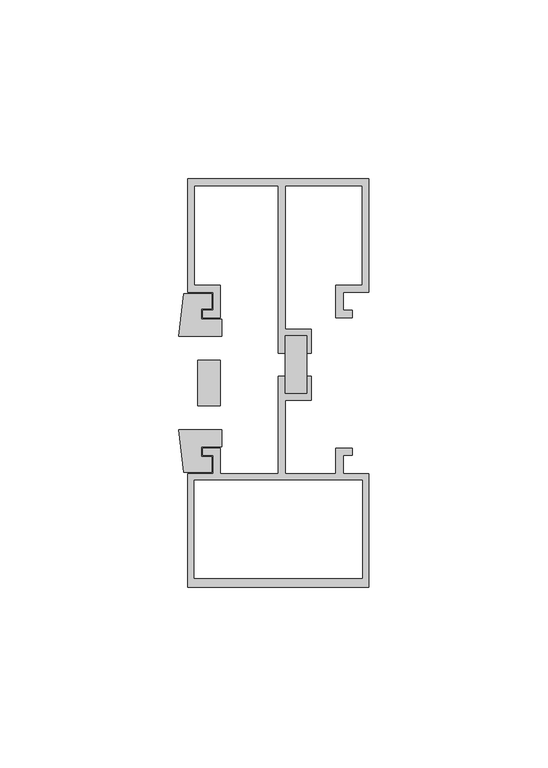
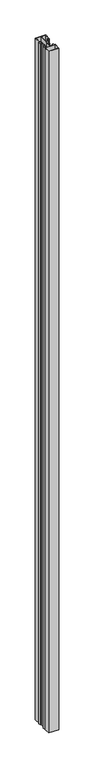
"""IFC4 building model written with IfcOpenShell, lengths in millimetres: proxy geometry, Generic Models 3:Generic Models 1:5:Generic Models 1:5 : Generic Models 3:Generic Models 1:300625:345888:Generic Models 1:5:Generic Models 1:5 : Generic Models 3:Generic Models 1:300625:345888 : Generic Models 3:Generic Models 1:5:Generic Models 1:5 : Generic Models 3:Generic Models 1:300625:345888:4 : Generic Models 3:Generic Models 1:5:Generic Models 1:5 : Generic Models 3:Generic Models 1:300625:345888:Generic Models 1:5:Generic Models 1:5 : Generic Models 3:Generic Models 1:300625:345888 : Generic Models 3:Generic Models 1:5:Generic Models 1:5 : Generic Models 3:Generic Models 1:300625:345888:301574."""

from ifc_helpers import new_model, si_unit, frame, origin, place, context, project, spatial, polyline, outline, extrude, source, transform, mapped, element, save


def generic_models_e0ac1aa3(model_context):
    return source(origin(), model_context, "Body", "SweptSolid", [
        extrude(outline(polyline([(570422.8035457, -579063.9802804), (570422.8035457, -579047.8688442), (570428.883333, -579047.8688442), (570428.883333, -579063.9802804), (570422.8035457, -579063.9802804)])), frame((0.0, 0.0, 66.3122056), z_axis=(0.0, 0.0, 1.0), x_axis=(1.0, 0.0, 0.0)), (0.0, 0.0, 1.0), 3584.971571),
        extrude(outline(polyline([(570398.3726303, -579067.3663841), (570398.3726303, -579054.6663841), (570404.7161787, -579054.6663841), (570404.7161787, -579067.3663841), (570398.3726303, -579067.3663841)])), frame((0.0, 0.0, 66.3122056), z_axis=(0.0, 0.0, 1.0), x_axis=(1.0, 0.0, 0.0)), (0.0, 0.0, 1.0), 3584.971571),
        extrude(outline(polyline([(570399.3995131, -579078.8588708), (570399.3995131, -579081.704549), (570402.3433729, -579081.704549), (570402.3433729, -579086.0026208), (570394.5036635, -579086.0026208), (570393.0427966, -579074.1048149), (570405.1130537, -579074.1048149), (570405.1130537, -579078.8588708), (570399.3995131, -579078.8588708)])), frame((0.0, 0.0, 66.3122056), z_axis=(0.0, 0.0, 1.0), x_axis=(1.0, 0.0, 0.0)), (0.0, 0.0, 1.0), 3584.971571),
        extrude(outline(polyline([(570394.5036635, -579036.0301474), (570402.3433729, -579036.0301474), (570402.3433729, -579040.3282192), (570399.3995131, -579040.3282192), (570399.3995131, -579043.1738974), (570405.1130537, -579043.1738974), (570405.1130537, -579047.9279532), (570393.0427966, -579047.9279532), (570394.5036635, -579036.0301474)])), frame((0.0, 0.0, 66.3122056), z_axis=(0.0, 0.0, 1.0), x_axis=(1.0, 0.0, 0.0)), (0.0, 0.0, 1.0), 3584.9377944),
        extrude(outline(polyline([(570446.2867239, -579118.1663841), (570395.5205005, -579118.1663841), (570395.5205005, -579086.3994958), (570402.7402479, -579086.3994958), (570402.7402479, -579081.307674), (570399.7963881, -579081.307674), (570399.7963881, -579079.2557458), (570404.7161787, -579079.2557458), (570404.7161787, -579086.3994958), (570420.9036122, -579086.3994958), (570420.9036122, -579059.1164506), (570422.8035457, -579059.1164506), (570422.8035457, -579063.9802804), (570428.883333, -579063.9802804), (570428.883333, -579059.1164506), (570430.1752878, -579059.1164506), (570430.1752878, -579065.8802139), (570422.8035457, -579065.8802139), (570422.8035457, -579086.3994958), (570437.0150484, -579086.3994958), (570437.0150484, -579079.2557458), (570441.586208, -579079.2557458), (570441.586208, -579081.307674), (570439.0669766, -579081.307674), (570439.0669766, -579086.3994958), (570446.2867239, -579086.3994958), (570446.2867239, -579118.1663841)]), holes=[polyline([(570397.420434, -579088.2994293), (570397.420434, -579115.6584719), (570444.3867904, -579115.6584719), (570444.3867904, -579088.2994293), (570397.420434, -579088.2994293)])]), frame((0.0, 0.0, 66.3122056), z_axis=(0.0, 0.0, 1.0), x_axis=(1.0, 0.0, 0.0)), (0.0, 0.0, 1.0), 3584.971571),
        extrude(outline(polyline([(570399.7963881, -579040.7250942), (570402.7402479, -579040.7250942), (570402.7402479, -579035.6332724), (570395.5205005, -579035.6332724), (570395.5205005, -579003.8663841), (570446.2867239, -579003.8663841), (570446.2867239, -579035.6332724), (570439.0669766, -579035.6332724), (570439.0669766, -579040.7250942), (570441.586208, -579040.7250942), (570441.586208, -579042.7770224), (570437.0150484, -579042.7770224), (570437.0150484, -579033.7333389), (570444.3645113, -579033.7333389), (570444.3645113, -579005.8423149), (570422.8035457, -579005.8423149), (570422.8035457, -579045.9689107), (570430.1752878, -579045.9689107), (570430.1752878, -579052.732674), (570428.883333, -579052.732674), (570428.883333, -579047.8688442), (570422.8035457, -579047.8688442), (570422.8035457, -579052.732674), (570420.9036122, -579052.732674), (570420.9036122, -579005.8423149), (570397.4302996, -579005.8423149), (570397.4302996, -579033.7333389), (570404.7161787, -579033.7333389), (570404.7161787, -579042.7770224), (570399.7963881, -579042.7770224), (570399.7963881, -579040.7250942)])), frame((0.0, 0.0, 66.3122056), z_axis=(0.0, 0.0, 1.0), x_axis=(1.0, 0.0, 0.0)), (0.0, 0.0, 1.0), 3584.971571),
    ])


if __name__ == "__main__":
    model = new_model("IFC4")
    model_context = context("Model", 3, world=origin())
    ifc_project = project(units=[si_unit("LENGTHUNIT", "METRE", prefix="MILLI")], contexts=[model_context])
    site = spatial("IfcSite", under=ifc_project)
    building = spatial("IfcBuilding", under=site)
    placement = place(None, origin())
    generic_models_shape = generic_models_e0ac1aa3(model_context)
    element("IfcBuildingElementProxy", 1, Name="Generic Models 3:Generic Models 1:5:Generic Models 1:5 : Generic Models 3:Generic Models 1:300625:345888:Generic Models 1:5:Generic Models 1:5 : Generic Models 3:Generic Models 1:300625:345888 : Generic Models 3:Generic Models 1:5:Generic Models 1:5 : Generic Models 3:Generic Models 1:300625:345888:4 : Generic Models 3:Generic Models 1:5:Generic Models 1:5 : Generic Models 3:Generic Models 1:300625:345888:Generic Models 1:5:Generic Models 1:5 : Generic Models 3:Generic Models 1:300625:345888 : Generic Models 3:Generic Models 1:5:Generic Models 1:5 : Generic Models 3:Generic Models 1:300625:345888:301574", ObjectType="Generic Models 3:Generic Models 1:5:Generic Models 1:5 : Generic Models 3:Generic Models 1:300625:345888:Generic Models 1:5:Generic Models 1:5 : Generic Models 3:Generic Models 1:300625:345888 : Generic Models 3:Generic Models 1:5:Generic Models 1:5 : Generic Models 3:Generic Models 1:300625:345888:4 : Generic Models 3:Generic Models 1:5:Generic Models 1:5 : Generic Models 3:Generic Models 1:300625:345888:Generic Models 1:5:Generic Models 1:5 : Generic Models 3:Generic Models 1:300625:345888 : Generic Models 3:Generic Models 1:5:Generic Models 1:5 : Generic Models 3:Generic Models 1:300625:345888:301574", at=placement, inside=building, context=model_context, shape_type="MappedRepresentation", body=[
        mapped(generic_models_shape, transform((0.0, 0.0, 0.0), x_axis=(1.0, 0.0, 0.0), y_axis=(0.0, 1.0, 0.0), z_axis=(0.0, 0.0, 1.0))),
    ])
    save(model, "model.ifc")

# Revit data of these elements
# Type "Generic Models 3:Generic Models 1:5:Generic Models 1:5 : Generic Models 3:Generic Models 1:300625:345888:Generic Models 1:5:Generic Models 1:5 : Generic Models 3:Generic Models 1:300625:345888 : Generic Models 3:Generic Models 1:5:Generic Models 1:5 : Generic Models 3:Generic Models 1:300625:345888:4 : Generic Models 3:Generic Models 1:5:Generic Models 1:5 : Generic Models 3:Generic Models 1:300625:345888:Generic Models 1:5:Generic Models 1:5 : Generic Models 3:Generic Models 1:300625:345888 : Generic Models 3:Generic Models 1:5:Generic Models 1:5 : Generic Models 3:Generic Models 1:300625:345888:301574"
#   NameOverride = "Generic Models 3:Generic Models 1:5:Generic Models 1:5 : Generic Models 3:Generic Models 1:300625:345888:Generic Models 1:5:Generic Models 1:5 : Generic Models 3:Generic Models 1:300625:345888 : Generic Models 3:Generic Models 1:5:Generic Models 1:5 : Generic Models 3:Generic Models 1:300625:345888:301574"
#   ObjectTypeOverride = "Generic Models 1:5:Generic Models 1:5 : Generic Models 3:Generic Models 1:300625:345888 : Generic Models 3:Generic Models 1:5:Generic Models 1:5 : Generic Models 3:Generic Models 1:300625:345888"
#   Reference = "Generic Models 1"
#   Tag = "301574"
# Element 1 (IfcBuildingElementProxy, "Generic Models 3:Generic Models 1:5:Generic Models 1:5 : Generic Models 3:Generic Models 1:300625:345888:Generic Models 1:5:Generic Models 1:5 : Generic Models 3:Generic Models 1:300625:345888 : Generic Models 3:Generic Models 1:5:Generic Models 1:5 : Generic Models 3:Generic Models 1:300625:345888:4 : Generic Models 3:Generic Models 1:5:Generic Models 1:5 : Generic Models 3:Generic Models 1:300625:345888:Generic Models 1:5:Generic Models 1:5 : Generic Models 3:Generic Models 1:300625:345888 : Generic Models 3:Generic Models 1:5:Generic Models 1:5 : Generic Models 3:Generic Models 1:300625:345888:301574")
#   Materials on its faces: "THERMAL BROKEN ALUMINUM STOREFRONT"
# Materials
#   "THERMAL BROKEN ALUMINUM STOREFRONT": class "Unassigned", colour RGB 244 244 244, transparency 0, Cost = 0
